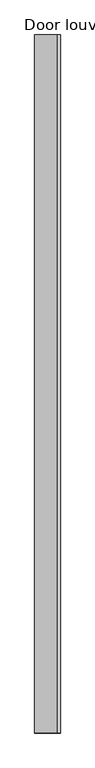
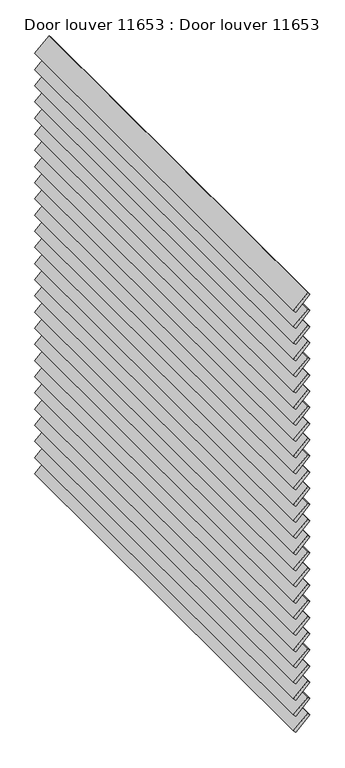
"""IFC4 building model written with IfcOpenShell, lengths in millimetres: proxy geometry, Door louver 11653 : Door louver 11653."""

from ifc_helpers import new_model, si_unit, frame, origin, place, context, project, spatial, polyline, outline, extrude, source, transform, mapped, element, save


def door_louver_11653_door_louver_11653_7676acec(model_context):
    return source(origin(), model_context, "Body", "SweptSolid", [
        extrude(outline(polyline([(0.0, -88.6), (0.0, 0.0), (2000.0, 0.0), (2000.0, -88.6), (0.0, -88.6)])), frame((-8304.3306423, 6540.4513244, 32854.8547367), z_axis=(-0.6925092278135618, 0.0, 0.721409016711785), x_axis=(0.0, -1.0, 0.0)), (0.0, 0.0, 1.0), 13.8216714),
        extrude(outline(polyline([(0.0, -88.6), (0.0, 0.0), (2000.0, 0.0), (2000.0, -88.6), (0.0, -88.6)])), frame((-8304.3306423, 6540.4513244, 32931.0547367), z_axis=(-0.6925092278135618, 0.0, 0.721409016711785), x_axis=(0.0, -1.0, 0.0)), (0.0, 0.0, 1.0), 13.8216714),
        extrude(outline(polyline([(0.0, -88.6), (0.0, 0.0), (2000.0, 0.0), (2000.0, -88.6), (0.0, -88.6)])), frame((-8304.3306423, 6540.4513244, 33007.2547367), z_axis=(-0.6925092278135618, 0.0, 0.721409016711785), x_axis=(0.0, -1.0, 0.0)), (0.0, 0.0, 1.0), 13.8216714),
        extrude(outline(polyline([(0.0, -88.6), (0.0, 0.0), (2000.0, 0.0), (2000.0, -88.6), (0.0, -88.6)])), frame((-8304.3306423, 6540.4513244, 33083.4547367), z_axis=(-0.6925092278135618, 0.0, 0.721409016711785), x_axis=(0.0, -1.0, 0.0)), (0.0, 0.0, 1.0), 13.8216714),
        extrude(outline(polyline([(0.0, -88.6), (0.0, 0.0), (2000.0, 0.0), (2000.0, -88.6), (0.0, -88.6)])), frame((-8304.3306423, 6540.4513244, 33159.6547367), z_axis=(-0.6925092278135618, 0.0, 0.721409016711785), x_axis=(0.0, -1.0, 0.0)), (0.0, 0.0, 1.0), 13.8216714),
        extrude(outline(polyline([(0.0, -88.6), (0.0, 0.0), (2000.0, 0.0), (2000.0, -88.6), (0.0, -88.6)])), frame((-8304.3306423, 6540.4513244, 33235.8547367), z_axis=(-0.6925092278135618, 0.0, 0.721409016711785), x_axis=(0.0, -1.0, 0.0)), (0.0, 0.0, 1.0), 13.8216714),
        extrude(outline(polyline([(0.0, -88.6), (0.0, 0.0), (2000.0, 0.0), (2000.0, -88.6), (0.0, -88.6)])), frame((-8304.3306423, 6540.4513244, 33312.0547367), z_axis=(-0.6925092278135618, 0.0, 0.721409016711785), x_axis=(0.0, -1.0, 0.0)), (0.0, 0.0, 1.0), 13.8216714),
        extrude(outline(polyline([(0.0, -88.6), (0.0, 0.0), (2000.0, 0.0), (2000.0, -88.6), (0.0, -88.6)])), frame((-8304.3306423, 6540.4513244, 33388.2547367), z_axis=(-0.6925092278135618, 0.0, 0.721409016711785), x_axis=(0.0, -1.0, 0.0)), (0.0, 0.0, 1.0), 13.8216714),
        extrude(outline(polyline([(0.0, -88.6), (0.0, 0.0), (2000.0, 0.0), (2000.0, -88.6), (0.0, -88.6)])), frame((-8304.3306423, 6540.4513244, 33464.4547367), z_axis=(-0.6925092278135618, 0.0, 0.721409016711785), x_axis=(0.0, -1.0, 0.0)), (0.0, 0.0, 1.0), 13.8216714),
        extrude(outline(polyline([(0.0, -88.6), (0.0, 0.0), (2000.0, 0.0), (2000.0, -88.6), (0.0, -88.6)])), frame((-8304.3306423, 6540.4513244, 33540.6547367), z_axis=(-0.6925092278135618, 0.0, 0.721409016711785), x_axis=(0.0, -1.0, 0.0)), (0.0, 0.0, 1.0), 13.8216714),
        extrude(outline(polyline([(0.0, -88.6), (0.0, 0.0), (2000.0, 0.0), (2000.0, -88.6), (0.0, -88.6)])), frame((-8304.3306423, 6540.4513244, 33616.8547367), z_axis=(-0.6925092278135618, 0.0, 0.721409016711785), x_axis=(0.0, -1.0, 0.0)), (0.0, 0.0, 1.0), 13.8216714),
        extrude(outline(polyline([(0.0, -88.6), (0.0, 0.0), (2000.0, 0.0), (2000.0, -88.6), (0.0, -88.6)])), frame((-8304.3306423, 6540.4513244, 33693.0547367), z_axis=(-0.6925092278135618, 0.0, 0.721409016711785), x_axis=(0.0, -1.0, 0.0)), (0.0, 0.0, 1.0), 13.8216714),
        extrude(outline(polyline([(0.0, -88.6), (0.0, 0.0), (2000.0, 0.0), (2000.0, -88.6), (0.0, -88.6)])), frame((-8304.3306423, 6540.4513244, 33769.2547367), z_axis=(-0.6925092278135618, 0.0, 0.721409016711785), x_axis=(0.0, -1.0, 0.0)), (0.0, 0.0, 1.0), 13.8216714),
        extrude(outline(polyline([(0.0, -88.6), (0.0, 0.0), (2000.0, 0.0), (2000.0, -88.6), (0.0, -88.6)])), frame((-8304.3306423, 6540.4513244, 33845.4547367), z_axis=(-0.6925092278135618, 0.0, 0.721409016711785), x_axis=(0.0, -1.0, 0.0)), (0.0, 0.0, 1.0), 13.8216714),
        extrude(outline(polyline([(0.0, -88.6), (0.0, 0.0), (2000.0, 0.0), (2000.0, -88.6), (0.0, -88.6)])), frame((-8304.3306423, 6540.4513244, 33921.6547367), z_axis=(-0.6925092278135618, 0.0, 0.721409016711785), x_axis=(0.0, -1.0, 0.0)), (0.0, 0.0, 1.0), 13.8216714),
        extrude(outline(polyline([(0.0, -88.6), (0.0, 0.0), (2000.0, 0.0), (2000.0, -88.6), (0.0, -88.6)])), frame((-8304.3306423, 6540.4513244, 33997.8547367), z_axis=(-0.6925092278135618, 0.0, 0.721409016711785), x_axis=(0.0, -1.0, 0.0)), (0.0, 0.0, 1.0), 13.8216714),
        extrude(outline(polyline([(0.0, -88.6), (0.0, 0.0), (2000.0, 0.0), (2000.0, -88.6), (0.0, -88.6)])), frame((-8304.3306423, 6540.4513244, 34074.0547367), z_axis=(-0.6925092278135618, 0.0, 0.721409016711785), x_axis=(0.0, -1.0, 0.0)), (0.0, 0.0, 1.0), 13.8216714),
        extrude(outline(polyline([(0.0, -88.6), (0.0, 0.0), (2000.0, 0.0), (2000.0, -88.6), (0.0, -88.6)])), frame((-8304.3306423, 6540.4513244, 34150.2547367), z_axis=(-0.6925092278135618, 0.0, 0.721409016711785), x_axis=(0.0, -1.0, 0.0)), (0.0, 0.0, 1.0), 13.8216714),
        extrude(outline(polyline([(0.0, -88.6), (0.0, 0.0), (2000.0, 0.0), (2000.0, -88.6), (0.0, -88.6)])), frame((-8304.3306423, 6540.4513244, 34226.4547367), z_axis=(-0.6925092278135618, 0.0, 0.721409016711785), x_axis=(0.0, -1.0, 0.0)), (0.0, 0.0, 1.0), 13.8216714),
        extrude(outline(polyline([(0.0, -88.6), (0.0, 0.0), (2000.0, 0.0), (2000.0, -88.6), (0.0, -88.6)])), frame((-8304.3306423, 6540.4513244, 34302.6547367), z_axis=(-0.6925092278135618, 0.0, 0.721409016711785), x_axis=(0.0, -1.0, 0.0)), (0.0, 0.0, 1.0), 13.8216714),
        extrude(outline(polyline([(0.0, -88.6), (0.0, 0.0), (2000.0, 0.0), (2000.0, -88.6), (0.0, -88.6)])), frame((-8304.3306423, 6540.4513244, 34378.8547367), z_axis=(-0.6925092278135618, 0.0, 0.721409016711785), x_axis=(0.0, -1.0, 0.0)), (0.0, 0.0, 1.0), 13.8216714),
        extrude(outline(polyline([(0.0, -88.6), (0.0, 0.0), (2000.0, 0.0), (2000.0, -88.6), (0.0, -88.6)])), frame((-8304.3306423, 6540.4513244, 34455.0547367), z_axis=(-0.6925092278135618, 0.0, 0.721409016711785), x_axis=(0.0, -1.0, 0.0)), (0.0, 0.0, 1.0), 13.8216714),
        extrude(outline(polyline([(0.0, -88.6), (0.0, 0.0), (2000.0, 0.0), (2000.0, -88.6), (0.0, -88.6)])), frame((-8304.3306423, 6540.4513244, 34531.2547367), z_axis=(-0.6925092278135618, 0.0, 0.721409016711785), x_axis=(0.0, -1.0, 0.0)), (0.0, 0.0, 1.0), 13.8216714),
        extrude(outline(polyline([(0.0, -88.6), (0.0, 0.0), (2000.0, 0.0), (2000.0, -88.6), (0.0, -88.6)])), frame((-8304.3306423, 6540.4513244, 34607.4547367), z_axis=(-0.6925092278135618, 0.0, 0.721409016711785), x_axis=(0.0, -1.0, 0.0)), (0.0, 0.0, 1.0), 13.8216714),
        extrude(outline(polyline([(0.0, -88.6), (0.0, 0.0), (2000.0, 0.0), (2000.0, -88.6), (0.0, -88.6)])), frame((-8304.3306423, 6540.4513244, 34683.6547367), z_axis=(-0.6925092278135618, 0.0, 0.721409016711785), x_axis=(0.0, -1.0, 0.0)), (0.0, 0.0, 1.0), 13.8216714),
        extrude(outline(polyline([(0.0, -88.6), (0.0, 0.0), (2000.0, 0.0), (2000.0, -88.6), (0.0, -88.6)])), frame((-8304.3306423, 6540.4513244, 34759.8547367), z_axis=(-0.6925092278135618, 0.0, 0.721409016711785), x_axis=(0.0, -1.0, 0.0)), (0.0, 0.0, 1.0), 13.8216714),
        extrude(outline(polyline([(0.0, -88.6), (0.0, 0.0), (2000.0, 0.0), (2000.0, -88.6), (0.0, -88.6)])), frame((-8304.3306423, 6540.4513244, 34836.0547367), z_axis=(-0.6925092278135618, 0.0, 0.721409016711785), x_axis=(0.0, -1.0, 0.0)), (0.0, 0.0, 1.0), 13.8216714),
    ])


if __name__ == "__main__":
    model = new_model("IFC4")
    model_context = context("Model", 3, world=origin())
    ifc_project = project(units=[si_unit("LENGTHUNIT", "METRE", prefix="MILLI")], contexts=[model_context])
    site = spatial("IfcSite", under=ifc_project)
    building = spatial("IfcBuilding", under=site)
    placement = place(None, origin())
    door_louver_11653_door_louver_11653_shape = door_louver_11653_door_louver_11653_7676acec(model_context)
    element("IfcBuildingElementProxy", 1, Name="Door louver 11653 : Door louver 11653", ObjectType="Door louver 11653 : Door louver 11653", at=placement, inside=building, context=model_context, shape_type="MappedRepresentation", body=[
        mapped(door_louver_11653_door_louver_11653_shape, transform((0.0, 0.0, 0.0), x_axis=(1.0, 0.0, 0.0), y_axis=(0.0, 1.0, 0.0), z_axis=(0.0, 0.0, 1.0))),
    ])
    save(model, "model.ifc")

# Revit data of these elements
# Type "Door louver 11653 : Door louver 11653"
#   NameOverride = "Door louver"
# Element 1 (IfcBuildingElementProxy, "Door louver 11653 : Door louver 11653")
#   Materials on its faces: "WOODEN LOUVERS (SPEC T. B. D.)"
# Materials
#   "WOODEN LOUVERS (SPEC T. B. D.)": class "Unassigned", colour RGB 148 103 60, transparency 0, Cost = 0
